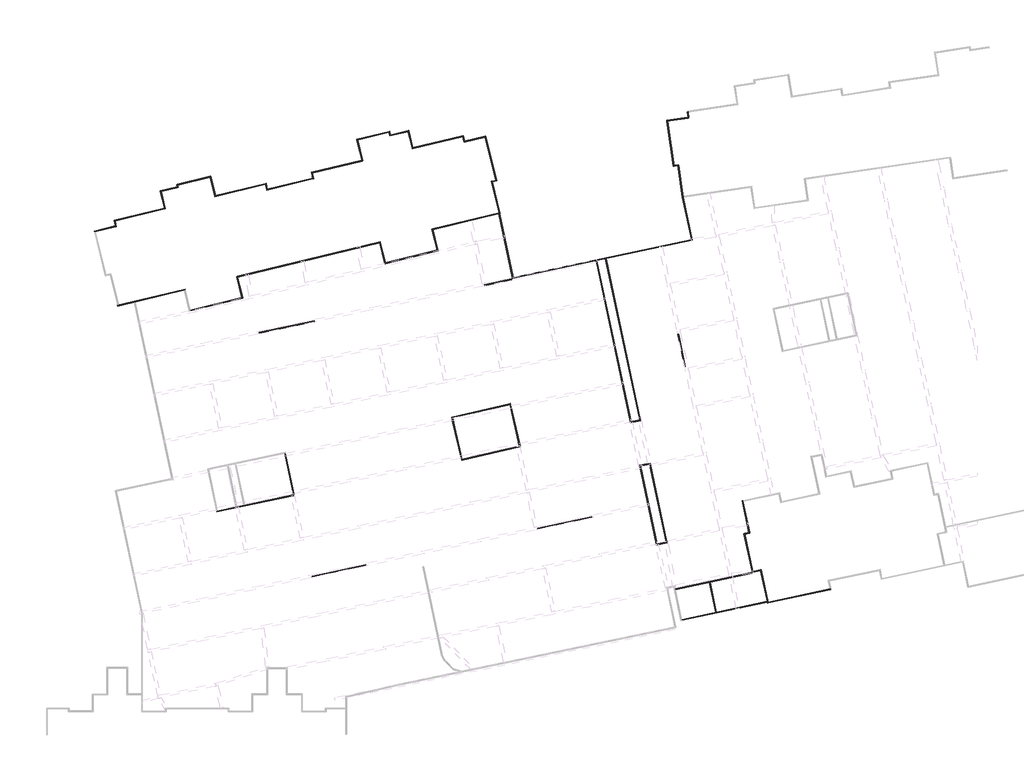
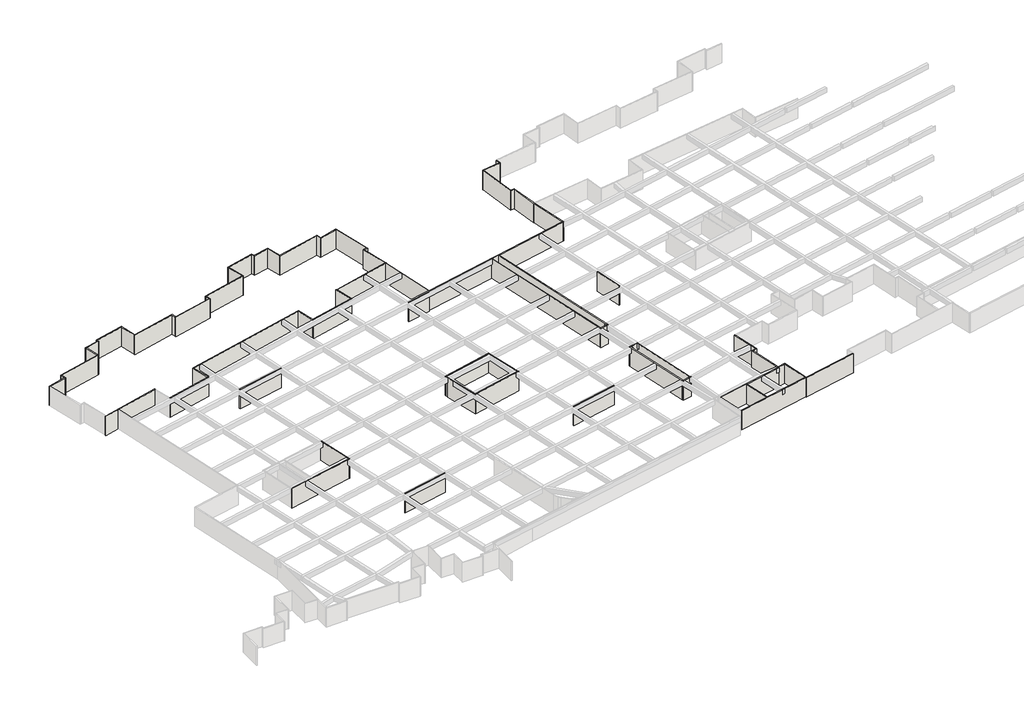
# One storey, part 2 of 14: 68 walls.
"""IFC4 building model written with IfcOpenShell, lengths in millimetres."""

from ifc_helpers import new_model, si_unit, origin, origin_with_axes, place, context, project, spatial, polyline, outline, extrude, faceted_brep, element, save

model = new_model("IFC4")

# Units and contexts
model_context = context("Model", 3, world=origin())
ifc_project = project(units=[si_unit("LENGTHUNIT", "METRE", prefix="MILLI")], contexts=[model_context])

# Site, building, storey
site = spatial("IfcSite", under=ifc_project)
building = spatial("IfcBuilding", under=site)
storey = spatial("IfcBuildingStorey", under=building, Name="户型图", Elevation=0.0)

# Walls
placement = place(None, origin())
element("IfcWall", 1, ObjectType="所有墙体", at=placement, inside=storey, context=model_context, shape_type="Brep", body=[
    faceted_brep([(-247680.1247195, -194264.9696016, 0.0), (-247705.0741224, -194147.5918895, 0.0), (-248661.634697, -189647.3282085, 0.0), (-248661.634697, -189647.3282085, 3300.0), (-247705.0741224, -194147.5918895, 3300.0), (-247680.1247195, -194264.9696016, 3300.0), (-247797.5024316, -194289.9190045, 0.0), (-247797.5024316, -194289.9190045, 3300.0), (-247821.8102949, -194175.5594989, 3300.0), (-247846.7596978, -194058.1817868, 3300.0), (-248754.0630062, -189789.6553235, 3300.0), (-248779.0124091, -189672.2776114, 3300.0), (-248779.0124091, -189672.2776114, 0.0), (-248754.0630062, -189789.6553235, 0.0), (-247846.7596978, -194058.1817868, 0.0), (-247821.8102949, -194175.5594989, 0.0)], [[[0, 1, 2, 3, 4, 5]], [[6, 7, 8, 9, 10, 11, 12, 13, 14, 15]], [[2, 1, 0, 6, 15, 14, 13, 12]], [[5, 4, 3, 11, 10, 9, 8, 7]], [[3, 2, 12, 11]], [[0, 5, 7, 6]]]),
])
element("IfcWall", 2, ObjectType="所有墙体", at=placement, inside=storey, context=model_context, shape_type="Brep", body=[
    faceted_brep([(-248779.0124091, -189672.2776114, 0.0), (-249835.4118179, -189896.8222375, 0.0), (-249952.78953, -189921.7716404, 0.0), (-249952.78953, -189921.7716404, 3300.0), (-249835.4118179, -189896.8222375, 3300.0), (-248779.0124091, -189672.2776114, 3300.0), (-248754.0630062, -189789.6553235, 0.0), (-248754.0630062, -189789.6553235, 3300.0), (-249927.8401271, -190039.1493525, 3300.0), (-249927.8401271, -190039.1493525, 0.0), (-249932.532469, -190017.0736194, 0.0), (-249932.532469, -190017.0736194, 3300.0)], [[[0, 1, 2, 3, 4, 5]], [[6, 7, 8, 9]], [[2, 1, 0, 6, 9, 10]], [[5, 4, 3, 11, 8, 7]], [[0, 5, 7, 6]], [[3, 2, 10, 9, 8, 11]]]),
])
element("IfcWall", 3, ObjectType="所有墙体", at=placement, inside=storey, context=model_context, shape_type="Brep", body=[
    faceted_brep([(-249835.4118179, -189896.8222375, 0.0), (-250933.1855454, -184732.2029056, 0.0), (-250958.1349483, -184614.8251935, 0.0), (-250958.1349483, -184614.8251935, 3300.0), (-250933.1855454, -184732.2029056, 3300.0), (-249835.4118179, -189896.8222375, 3300.0), (-249952.78953, -189921.7716404, 0.0), (-249952.78953, -189921.7716404, 3300.0), (-251075.5126604, -184639.7745964, 3300.0), (-251075.5126604, -184639.7745964, 0.0)], [[[0, 1, 2, 3, 4, 5]], [[6, 7, 8, 9]], [[2, 1, 0, 6, 9]], [[5, 4, 3, 8, 7]], [[0, 5, 7, 6]], [[3, 2, 9, 8]]]),
])
element("IfcWall", 4, ObjectType="所有墙体", at=placement, inside=storey, context=model_context, shape_type="Brep", body=[
    faceted_brep([(-250933.1855454, -184732.2029056, 0.0), (-250248.4822249, -184586.6647221, 0.0), (-250248.4822249, -184586.6647221, 3300.0), (-250933.1855454, -184732.2029056, 3300.0), (-250958.1349483, -184614.8251935, 0.0), (-250958.1349483, -184614.8251935, 3300.0), (-250390.8093399, -184494.2364129, 3300.0), (-250273.4316278, -184469.28701, 3300.0), (-250273.4316278, -184469.28701, 0.0), (-250390.8093399, -184494.2364129, 0.0)], [[[0, 1, 2, 3]], [[4, 5, 6, 7, 8, 9]], [[1, 0, 4, 9, 8]], [[3, 2, 7, 6, 5]], [[0, 3, 5, 4]], [[2, 1, 8, 7]]]),
])
element("IfcWall", 5, ObjectType="所有墙体", at=placement, inside=storey, context=model_context, shape_type="Brep", body=[
    faceted_brep([(-250273.4316278, -184469.28701, 0.0), (-251184.7932427, -180181.6677158, 0.0), (-251209.7426456, -180064.2900037, 0.0), (-251209.7426456, -180064.2900037, 3300.0), (-251184.7932427, -180181.6677158, 3300.0), (-250273.4316278, -184469.28701, 3300.0), (-250390.8093399, -184494.2364129, 0.0), (-250390.8093399, -184494.2364129, 3300.0), (-251327.1203577, -180089.2394066, 3300.0), (-251327.1203577, -180089.2394066, 0.0)], [[[0, 1, 2, 3, 4, 5]], [[6, 7, 8, 9]], [[2, 1, 0, 6, 9]], [[5, 4, 3, 8, 7]], [[0, 5, 7, 6]], [[3, 2, 9, 8]]]),
])
element("IfcWall", 6, ObjectType="所有墙体", at=placement, inside=storey, context=model_context, shape_type="SweptSolid", body=[
    extrude(outline(polyline([(-247705.0741224, -194147.5918895), (-239110.0463222, -192320.6623328), (-239085.0969193, -192438.0400449), (-247680.1247195, -194264.9696016), (-247705.0741224, -194147.5918895)])), origin_with_axes(), (0.0, 0.0, 1.0), 3300.0),
])
element("IfcWall", 7, ObjectType="所有墙体", at=placement, inside=storey, context=model_context, shape_type="Brep", body=[
    faceted_brep([(-258948.9869471, -126119.2790497, 0.0), (-258844.3642989, -126831.6371769, 0.0), (-258826.9271908, -126950.3635315, 0.0), (-258826.9271908, -126950.3635315, 3300.0), (-258844.3642989, -126831.6371769, 3300.0), (-258948.9869471, -126119.2790497, 3300.0), (-258830.2605925, -126101.8419416, 0.0), (-258830.2605925, -126101.8419416, 3300.0), (-258708.2008363, -126932.9264234, 3300.0), (-258708.2008363, -126932.9264234, 0.0)], [[[0, 1, 2, 3, 4, 5]], [[6, 7, 8, 9]], [[2, 1, 0, 6, 9]], [[5, 4, 3, 8, 7]], [[0, 5, 7, 6]], [[3, 2, 9, 8]]]),
])
element("IfcWall", 8, ObjectType="所有墙体", at=placement, inside=storey, context=model_context, shape_type="Brep", body=[
    faceted_brep([(-258844.3642989, -126831.6371769, 0.0), (-261812.5231625, -127267.5648778, 0.0), (-261812.5231625, -127267.5648778, 3300.0), (-258844.3642989, -126831.6371769, 3300.0), (-258826.9271908, -126950.3635315, 0.0), (-258826.9271908, -126950.3635315, 3300.0), (-261676.3596999, -127368.8541243, 3300.0), (-261795.0860545, -127386.2912323, 3300.0), (-261795.0860545, -127386.2912323, 0.0), (-261676.3596999, -127368.8541243, 0.0)], [[[0, 1, 2, 3]], [[4, 5, 6, 7, 8, 9]], [[1, 0, 4, 9, 8]], [[3, 2, 7, 6, 5]], [[0, 3, 5, 4]], [[2, 1, 8, 7]]]),
])
element("IfcWall", 9, ObjectType="所有墙体", at=placement, inside=storey, context=model_context, shape_type="Brep", body=[
    faceted_brep([(-261795.0860545, -127386.2912323, 0.0), (-260879.6378827, -133619.4248459, 0.0), (-260879.6378827, -133619.4248459, 3300.0), (-261795.0860545, -127386.2912323, 3300.0), (-261676.3596999, -127368.8541243, 0.0), (-261676.3596999, -127368.8541243, 3300.0), (-260778.3486362, -133483.2613833, 3300.0), (-260760.9115282, -133601.9877379, 3300.0), (-260760.9115282, -133601.9877379, 0.0), (-260778.3486362, -133483.2613833, 0.0)], [[[0, 1, 2, 3]], [[4, 5, 6, 7, 8, 9]], [[1, 0, 4, 9, 8]], [[3, 2, 7, 6, 5]], [[0, 3, 5, 4]], [[2, 1, 8, 7]]]),
])
element("IfcWall", 10, ObjectType="所有墙体", at=placement, inside=storey, context=model_context, shape_type="Brep", body=[
    faceted_brep([(-260760.9115282, -133601.9877379, 0.0), (-260267.9501372, -133529.5874602, 0.0), (-260149.2237827, -133512.1503522, 0.0), (-260149.2237827, -133512.1503522, 3300.0), (-260267.9501372, -133529.5874602, 3300.0), (-260760.9115282, -133601.9877379, 3300.0), (-260778.3486362, -133483.2613833, 0.0), (-260778.3486362, -133483.2613833, 3300.0), (-260166.6608907, -133393.4239977, 3300.0), (-260166.6608907, -133393.4239977, 0.0)], [[[0, 1, 2, 3, 4, 5]], [[6, 7, 8, 9]], [[2, 1, 0, 6, 9]], [[5, 4, 3, 8, 7]], [[0, 5, 7, 6]], [[3, 2, 9, 8]]]),
])
element("IfcWall", 11, ObjectType="所有墙体", at=placement, inside=storey, context=model_context, shape_type="Brep", body=[
    faceted_brep([(-260267.9501372, -133529.5874602, 0.0), (-259616.5559691, -137964.8214911, 0.0), (-259616.5559691, -137964.8214911, 3300.0), (-260267.9501372, -133529.5874602, 3300.0), (-260149.2237827, -133512.1503522, 0.0), (-260149.2237827, -133512.1503522, 3300.0), (-259515.2667226, -137828.6580286, 3300.0), (-259497.8296146, -137947.3843831, 3300.0), (-259497.8296146, -137947.3843831, 0.0), (-259515.2667226, -137828.6580286, 0.0), (-259612.8948547, -137964.2837904, 0.0), (-259612.8948547, -137964.2837904, 3300.0)], [[[0, 1, 2, 3]], [[4, 5, 6, 7, 8, 9]], [[1, 0, 4, 9, 8, 10]], [[3, 2, 11, 7, 6, 5]], [[0, 3, 5, 4]], [[2, 1, 10, 8, 7, 11]]]),
])
element("IfcWall", 12, ObjectType="所有墙体", at=placement, inside=storey, context=model_context, shape_type="Brep", body=[
    faceted_brep([(-338038.3860994, -153082.5880427, 0.0), (-335711.2604986, -152517.7311777, 0.0), (-335594.5985969, -152489.4141517, 0.0), (-328767.5797313, -150832.3104387, 0.0), (-328650.9658147, -150804.0050601, 0.0), (-328650.9658147, -150804.0050601, 3300.0), (-328767.5797313, -150832.3104387, 3300.0), (-335594.5985969, -152489.4141517, 3300.0), (-335711.2604986, -152517.7311777, 3300.0), (-338038.3860994, -153082.5880427, 3300.0), (-338066.691478, -152965.9741261, 0.0), (-338066.691478, -152965.9741261, 3300.0), (-338027.8201762, -152956.5390008, 3300.0), (-337911.2062596, -152928.2336221, 3300.0), (-328679.2711934, -150687.3911435, 3300.0), (-328679.2711934, -150687.3911435, 0.0), (-337911.2062596, -152928.2336221, 0.0), (-338027.8201762, -152956.5390008, 0.0)], [[[0, 1, 2, 3, 4, 5, 6, 7, 8, 9]], [[10, 11, 12, 13, 14, 15, 16, 17]], [[4, 3, 2, 1, 0, 10, 17, 16, 15]], [[9, 8, 7, 6, 5, 14, 13, 12, 11]], [[0, 9, 11, 10]], [[5, 4, 15, 14]]]),
])
element("IfcWall", 13, ObjectType="所有墙体", at=placement, inside=storey, context=model_context, shape_type="Brep", body=[
    faceted_brep([(-327943.3313501, -153719.3529662, 0.0), (-320654.9615625, -151950.2667992, 0.0), (-320654.9615625, -151950.2667992, 3300.0), (-327943.3313501, -153719.3529662, 3300.0), (-327971.6367288, -153602.7390496, 0.0), (-327971.6367288, -153602.7390496, 3300.0), (-320799.8808577, -151861.9582613, 3300.0), (-320683.2669411, -151833.6528826, 3300.0), (-320683.2669411, -151833.6528826, 0.0), (-320799.8808577, -151861.9582613, 0.0)], [[[0, 1, 2, 3]], [[4, 5, 6, 7, 8, 9]], [[1, 0, 4, 9, 8]], [[3, 2, 7, 6, 5]], [[0, 3, 5, 4]], [[2, 1, 8, 7]]]),
])
element("IfcWall", 14, ObjectType="所有墙体", at=placement, inside=storey, context=model_context, shape_type="Brep", body=[
    faceted_brep([(-320683.2669411, -151833.6528826, 0.0), (-321362.5960271, -149034.9188931, 0.0), (-321390.9014057, -148918.3049765, 0.0), (-321390.9014057, -148918.3049765, 3300.0), (-321362.5960271, -149034.9188931, 3300.0), (-320683.2669411, -151833.6528826, 3300.0), (-320799.8808577, -151861.9582613, 0.0), (-320799.8808577, -151861.9582613, 3300.0), (-321507.5153223, -148946.6103552, 3300.0), (-321507.5153223, -148946.6103552, 0.0)], [[[0, 1, 2, 3, 4, 5]], [[6, 7, 8, 9]], [[2, 1, 0, 6, 9]], [[5, 4, 3, 8, 7]], [[0, 5, 7, 6]], [[3, 2, 9, 8]]]),
])
element("IfcWall", 15, ObjectType="所有墙体", at=placement, inside=storey, context=model_context, shape_type="Brep", body=[
    faceted_brep([(-321362.5960271, -149034.9188931, 0.0), (-301654.8441261, -144251.3098988, 0.0), (-301538.2302095, -144223.0045201, 0.0), (-301538.2302095, -144223.0045201, 3300.0), (-301654.8441261, -144251.3098988, 3300.0), (-321362.5960271, -149034.9188931, 3300.0), (-321390.9014057, -148918.3049765, 0.0), (-321390.9014057, -148918.3049765, 3300.0), (-301566.5355882, -144106.3906035, 3300.0), (-301566.5355882, -144106.3906035, 0.0)], [[[0, 1, 2, 3, 4, 5]], [[6, 7, 8, 9]], [[2, 1, 0, 6, 9]], [[5, 4, 3, 8, 7]], [[0, 5, 7, 6]], [[3, 2, 9, 8]]]),
])
element("IfcWall", 16, ObjectType="所有墙体", at=placement, inside=storey, context=model_context, shape_type="Brep", body=[
    faceted_brep([(-301654.8441261, -144251.3098988, 0.0), (-300947.2096643, -147166.6577934, 0.0), (-300947.2096643, -147166.6577934, 3300.0), (-301654.8441261, -144251.3098988, 3300.0), (-301538.2302095, -144223.0045201, 0.0), (-301538.2302095, -144223.0045201, 3300.0), (-300858.9011264, -147021.7384982, 3300.0), (-300830.5957477, -147138.3524148, 3300.0), (-300830.5957477, -147138.3524148, 0.0), (-300858.9011264, -147021.7384982, 0.0)], [[[0, 1, 2, 3]], [[4, 5, 6, 7, 8, 9]], [[1, 0, 4, 9, 8]], [[3, 2, 7, 6, 5]], [[0, 3, 5, 4]], [[2, 1, 8, 7]]]),
])
element("IfcWall", 17, ObjectType="所有墙体", at=placement, inside=storey, context=model_context, shape_type="Brep", body=[
    faceted_brep([(-300830.5957477, -147138.3524148, 0.0), (-293542.2259606, -145369.2662479, 0.0), (-293542.2259606, -145369.2662479, 3300.0), (-300830.5957477, -147138.3524148, 3300.0), (-300858.9011264, -147021.7384982, 0.0), (-300858.9011264, -147021.7384982, 3300.0), (-293687.1452559, -145280.95771, 3300.0), (-293570.5313393, -145252.6523314, 3300.0), (-293570.5313393, -145252.6523314, 0.0), (-293687.1452559, -145280.95771, 0.0)], [[[0, 1, 2, 3]], [[4, 5, 6, 7, 8, 9]], [[1, 0, 4, 9, 8]], [[3, 2, 7, 6, 5]], [[0, 3, 5, 4]], [[2, 1, 8, 7]]]),
])
element("IfcWall", 18, ObjectType="所有墙体", at=placement, inside=storey, context=model_context, shape_type="Brep", body=[
    faceted_brep([(-293570.5313393, -145252.6523314, 0.0), (-294249.8604225, -142453.9183533, 0.0), (-294278.1658011, -142337.3044367, 0.0), (-294278.1658011, -142337.3044367, 3300.0), (-294249.8604225, -142453.9183533, 3300.0), (-293570.5313393, -145252.6523314, 3300.0), (-293687.1452559, -145280.95771, 0.0), (-293687.1452559, -145280.95771, 3300.0), (-294394.7797177, -142365.6098154, 3300.0), (-294394.7797177, -142365.6098154, 0.0)], [[[0, 1, 2, 3, 4, 5]], [[6, 7, 8, 9]], [[2, 1, 0, 6, 9]], [[5, 4, 3, 8, 7]], [[0, 5, 7, 6]], [[3, 2, 9, 8]]]),
])
element("IfcWall", 19, ObjectType="所有墙体", at=placement, inside=storey, context=model_context, shape_type="Brep", body=[
    faceted_brep([(-294249.8604225, -142453.9183533, 0.0), (-285098.2083864, -140232.5627561, 0.0), (-284981.5464847, -140204.2457302, 0.0), (-284920.7470789, -140189.4880558, 0.0), (-284920.7470789, -140189.4880558, 3300.0), (-284981.5464847, -140204.2457302, 3300.0), (-285098.2083864, -140232.5627561, 3300.0), (-294249.8604225, -142453.9183533, 3300.0), (-294278.1658011, -142337.3044367, 0.0), (-294278.1658011, -142337.3044367, 3300.0), (-285065.6663741, -140101.1795179, 3300.0), (-284949.0524575, -140072.8741393, 3300.0), (-284949.0524575, -140072.8741393, 0.0), (-285065.6663741, -140101.1795179, 0.0)], [[[0, 1, 2, 3, 4, 5, 6, 7]], [[8, 9, 10, 11, 12, 13]], [[3, 2, 1, 0, 8, 13, 12]], [[7, 6, 5, 4, 11, 10, 9]], [[0, 7, 9, 8]], [[4, 3, 12, 11]]]),
])
element("IfcWall", 20, ObjectType="所有墙体", at=placement, inside=storey, context=model_context, shape_type="Brep", body=[
    faceted_brep([(-284949.0524575, -140072.8741393, 0.0), (-285982.1987791, -135816.4661828, 0.0), (-286010.5041578, -135699.8522663, 0.0), (-286010.5041578, -135699.8522663, 3300.0), (-285982.1987791, -135816.4661828, 3300.0), (-284949.0524575, -140072.8741393, 3300.0), (-285065.6663741, -140101.1795179, 0.0), (-285065.6663741, -140101.1795179, 3300.0), (-286127.1180744, -135728.1576449, 3300.0), (-286127.1180744, -135728.1576449, 0.0)], [[[0, 1, 2, 3, 4, 5]], [[6, 7, 8, 9]], [[2, 1, 0, 6, 9]], [[5, 4, 3, 8, 7]], [[0, 5, 7, 6]], [[3, 2, 9, 8]]]),
])
element("IfcWall", 21, ObjectType="所有墙体", at=placement, inside=storey, context=model_context, shape_type="Brep", body=[
    faceted_brep([(-285982.1987791, -135816.4661828, 0.0), (-285399.1292138, -135674.9392938, 0.0), (-285399.1292138, -135674.9392938, 3300.0), (-285982.1987791, -135816.4661828, 3300.0), (-286010.5041578, -135699.8522663, 0.0), (-286010.5041578, -135699.8522663, 3300.0), (-285544.0485091, -135586.6307559, 3300.0), (-285427.4345925, -135558.3253772, 3300.0), (-285427.4345925, -135558.3253772, 0.0), (-285544.0485091, -135586.6307559, 0.0)], [[[0, 1, 2, 3]], [[4, 5, 6, 7, 8, 9]], [[1, 0, 4, 9, 8]], [[3, 2, 7, 6, 5]], [[0, 3, 5, 4]], [[2, 1, 8, 7]]]),
])
element("IfcWall", 22, ObjectType="所有墙体", at=placement, inside=storey, context=model_context, shape_type="Brep", body=[
    faceted_brep([(-285427.4345925, -135558.3253772, 0.0), (-286913.4669714, -129436.0947611, 0.0), (-286913.4669714, -129436.0947611, 3300.0), (-285427.4345925, -135558.3253772, 3300.0), (-285544.0485091, -135586.6307559, 0.0), (-285544.0485091, -135586.6307559, 3300.0), (-287001.7755093, -129581.0140564, 3300.0), (-287030.080888, -129464.4001398, 3300.0), (-287030.080888, -129464.4001398, 0.0), (-287001.7755093, -129581.0140564, 0.0)], [[[0, 1, 2, 3]], [[4, 5, 6, 7, 8, 9]], [[1, 0, 4, 9, 8]], [[3, 2, 7, 6, 5]], [[0, 3, 5, 4]], [[2, 1, 8, 7]]]),
])
element("IfcWall", 23, ObjectType="所有墙体", at=placement, inside=storey, context=model_context, shape_type="Brep", body=[
    faceted_brep([(-287030.080888, -129464.4001398, 0.0), (-289828.8148854, -130143.7292277, 0.0), (-289945.428802, -130172.0346063, 0.0), (-289945.428802, -130172.0346063, 3300.0), (-289828.8148854, -130143.7292277, 3300.0), (-287030.080888, -129464.4001398, 3300.0), (-287001.7755093, -129581.0140564, 0.0), (-287001.7755093, -129581.0140564, 3300.0), (-289917.1234233, -130288.6485229, 3300.0), (-289917.1234233, -130288.6485229, 0.0)], [[[0, 1, 2, 3, 4, 5]], [[6, 7, 8, 9]], [[2, 1, 0, 6, 9]], [[5, 4, 3, 8, 7]], [[0, 5, 7, 6]], [[3, 2, 9, 8]]]),
])
element("IfcWall", 24, ObjectType="所有墙体", at=placement, inside=storey, context=model_context, shape_type="Brep", body=[
    faceted_brep([(-289828.8148854, -130143.7292277, 0.0), (-290017.5174109, -129366.3031131, 0.0), (-290017.5174109, -129366.3031131, 3300.0), (-289828.8148854, -130143.7292277, 3300.0), (-289945.428802, -130172.0346063, 0.0), (-289945.428802, -130172.0346063, 3300.0), (-290105.8259488, -129511.2224083, 3300.0), (-290134.1313274, -129394.6084918, 3300.0), (-290134.1313274, -129394.6084918, 0.0), (-290105.8259488, -129511.2224083, 0.0)], [[[0, 1, 2, 3]], [[4, 5, 6, 7, 8, 9]], [[1, 0, 4, 9, 8]], [[3, 2, 7, 6, 5]], [[0, 3, 5, 4]], [[2, 1, 8, 7]]]),
])
element("IfcWall", 25, ObjectType="所有墙体", at=placement, inside=storey, context=model_context, shape_type="Brep", body=[
    faceted_brep([(-290134.1313274, -129394.6084918, 0.0), (-297038.6469685, -131070.5227862, 0.0), (-297155.260885, -131098.8281648, 0.0), (-297155.260885, -131098.8281648, 3300.0), (-297038.6469685, -131070.5227862, 3300.0), (-290134.1313274, -129394.6084918, 3300.0), (-290105.8259488, -129511.2224083, 0.0), (-290105.8259488, -129511.2224083, 3300.0), (-297126.9555064, -131215.4420814, 3300.0), (-297126.9555064, -131215.4420814, 0.0)], [[[0, 1, 2, 3, 4, 5]], [[6, 7, 8, 9]], [[2, 1, 0, 6, 9]], [[5, 4, 3, 8, 7]], [[0, 5, 7, 6]], [[3, 2, 9, 8]]]),
])
element("IfcWall", 26, ObjectType="所有墙体", at=placement, inside=storey, context=model_context, shape_type="Brep", body=[
    faceted_brep([(-297038.6469685, -131070.5227862, 0.0), (-297622.4454055, -128665.3607481, 0.0), (-297622.4454055, -128665.3607481, 3300.0), (-297038.6469685, -131070.5227862, 3300.0), (-297155.260885, -131098.8281648, 0.0), (-297155.260885, -131098.8281648, 3300.0), (-297710.7539434, -128810.2800434, 3300.0), (-297739.0593221, -128693.6661268, 3300.0), (-297739.0593221, -128693.6661268, 0.0), (-297710.7539434, -128810.2800434, 0.0)], [[[0, 1, 2, 3]], [[4, 5, 6, 7, 8, 9]], [[1, 0, 4, 9, 8]], [[3, 2, 7, 6, 5]], [[0, 3, 5, 4]], [[2, 1, 8, 7]]]),
])
element("IfcWall", 27, ObjectType="所有墙体", at=placement, inside=storey, context=model_context, shape_type="Brep", body=[
    faceted_brep([(-297739.0593221, -128693.6661268, 0.0), (-300149.0802646, -129278.6439525, 0.0), (-300265.6941812, -129306.9493312, 0.0), (-300265.6941812, -129306.9493312, 3300.0), (-300149.0802646, -129278.6439525, 3300.0), (-297739.0593221, -128693.6661268, 3300.0), (-297710.7539434, -128810.2800434, 0.0), (-297710.7539434, -128810.2800434, 3300.0), (-300237.3888025, -129423.5632478, 3300.0), (-300237.3888025, -129423.5632478, 0.0)], [[[0, 1, 2, 3, 4, 5]], [[6, 7, 8, 9]], [[2, 1, 0, 6, 9]], [[5, 4, 3, 8, 7]], [[0, 5, 7, 6]], [[3, 2, 9, 8]]]),
])
element("IfcWall", 28, ObjectType="所有墙体", at=placement, inside=storey, context=model_context, shape_type="Brep", body=[
    faceted_brep([(-300149.0802646, -129278.6439525, 0.0), (-300267.0193424, -128792.7526335, 0.0), (-300267.0193424, -128792.7526335, 3300.0), (-300149.0802646, -129278.6439525, 3300.0), (-300265.6941812, -129306.9493312, 0.0), (-300265.6941812, -129306.9493312, 3300.0), (-300355.3278803, -128937.6719287, 3300.0), (-300383.633259, -128821.0580121, 3300.0), (-300383.633259, -128821.0580121, 0.0), (-300355.3278803, -128937.6719287, 0.0)], [[[0, 1, 2, 3]], [[4, 5, 6, 7, 8, 9]], [[1, 0, 4, 9, 8]], [[3, 2, 7, 6, 5]], [[0, 3, 5, 4]], [[2, 1, 8, 7]]]),
])
element("IfcWall", 29, ObjectType="所有墙体", at=placement, inside=storey, context=model_context, shape_type="Brep", body=[
    faceted_brep([(-300383.633259, -128821.0580121, 0.0), (-304829.5388252, -129900.200573, 0.0), (-304829.5388252, -129900.200573, 3300.0), (-300383.633259, -128821.0580121, 3300.0), (-300355.3278803, -128937.6719287, 0.0), (-300355.3278803, -128937.6719287, 3300.0), (-304684.61953, -129988.5091109, 3300.0), (-304801.2334465, -130016.8144895, 3300.0), (-304801.2334465, -130016.8144895, 0.0), (-304684.61953, -129988.5091109, 0.0)], [[[0, 1, 2, 3]], [[4, 5, 6, 7, 8, 9]], [[1, 0, 4, 9, 8]], [[3, 2, 7, 6, 5]], [[0, 3, 5, 4]], [[2, 1, 8, 7]]]),
])
element("IfcWall", 30, ObjectType="所有墙体", at=placement, inside=storey, context=model_context, shape_type="Brep", body=[
    faceted_brep([(-304801.2334465, -130016.8144895, 0.0), (-304127.8013104, -132791.2539301, 0.0), (-304099.4959317, -132907.8678466, 0.0), (-304099.4959317, -132907.8678466, 3300.0), (-304127.8013104, -132791.2539301, 3300.0), (-304801.2334465, -130016.8144895, 3300.0), (-304684.61953, -129988.5091109, 0.0), (-304684.61953, -129988.5091109, 3300.0), (-303982.8820151, -132879.562468, 3300.0), (-303982.8820151, -132879.562468, 0.0)], [[[0, 1, 2, 3, 4, 5]], [[6, 7, 8, 9]], [[2, 1, 0, 6, 9]], [[5, 4, 3, 8, 7]], [[0, 5, 7, 6]], [[3, 2, 9, 8]]]),
])
element("IfcWall", 31, ObjectType="所有墙体", at=placement, inside=storey, context=model_context, shape_type="Brep", body=[
    faceted_brep([(-304127.8013104, -132791.2539301, 0.0), (-311124.6363112, -134489.5766515, 0.0), (-311124.6363112, -134489.5766515, 3300.0), (-304127.8013104, -132791.2539301, 3300.0), (-304099.4959317, -132907.8678466, 0.0), (-304099.4959317, -132907.8678466, 3300.0), (-310979.7170159, -134577.8851894, 3300.0), (-311096.3309325, -134606.1905681, 3300.0), (-311096.3309325, -134606.1905681, 0.0), (-310979.7170159, -134577.8851894, 0.0)], [[[0, 1, 2, 3]], [[4, 5, 6, 7, 8, 9]], [[1, 0, 4, 9, 8]], [[3, 2, 7, 6, 5]], [[0, 3, 5, 4]], [[2, 1, 8, 7]]]),
])
element("IfcWall", 32, ObjectType="所有墙体", at=placement, inside=storey, context=model_context, shape_type="Brep", body=[
    faceted_brep([(-311096.3309325, -134606.1905681, 0.0), (-310935.933787, -135267.0027608, 0.0), (-310907.6284084, -135383.6166773, 0.0), (-310907.6284084, -135383.6166773, 3300.0), (-310935.933787, -135267.0027608, 3300.0), (-311096.3309325, -134606.1905681, 3300.0), (-310979.7170159, -134577.8851894, 0.0), (-310979.7170159, -134577.8851894, 3300.0), (-310791.0144918, -135355.3112987, 3300.0), (-310791.0144918, -135355.3112987, 0.0)], [[[0, 1, 2, 3, 4, 5]], [[6, 7, 8, 9]], [[2, 1, 0, 6, 9]], [[5, 4, 3, 8, 7]], [[0, 5, 7, 6]], [[3, 2, 9, 8]]]),
])
element("IfcWall", 33, ObjectType="所有墙体", at=placement, inside=storey, context=model_context, shape_type="Brep", body=[
    faceted_brep([(-310935.933787, -135267.0027608, 0.0), (-317233.0852904, -136795.4932107, 0.0), (-317349.699207, -136823.7985893, 0.0), (-317349.699207, -136823.7985893, 3300.0), (-317233.0852904, -136795.4932107, 3300.0), (-310935.933787, -135267.0027608, 3300.0), (-310907.6284084, -135383.6166773, 0.0), (-310907.6284084, -135383.6166773, 3300.0), (-317321.3938283, -136940.4125059, 3300.0), (-317321.3938283, -136940.4125059, 0.0)], [[[0, 1, 2, 3, 4, 5]], [[6, 7, 8, 9]], [[2, 1, 0, 6, 9]], [[5, 4, 3, 8, 7]], [[0, 5, 7, 6]], [[3, 2, 9, 8]]]),
])
element("IfcWall", 34, ObjectType="所有墙体", at=placement, inside=storey, context=model_context, shape_type="Brep", body=[
    faceted_brep([(-317233.0852904, -136795.4932107, 0.0), (-317421.7878145, -136018.0671014, 0.0), (-317421.7878145, -136018.0671014, 3300.0), (-317233.0852904, -136795.4932107, 3300.0), (-317349.699207, -136823.7985893, 0.0), (-317349.699207, -136823.7985893, 3300.0), (-317510.0963524, -136162.9863966, 3300.0), (-317538.4017311, -136046.3724801, 3300.0), (-317538.4017311, -136046.3724801, 0.0), (-317510.0963524, -136162.9863966, 0.0)], [[[0, 1, 2, 3]], [[4, 5, 6, 7, 8, 9]], [[1, 0, 4, 9, 8]], [[3, 2, 7, 6, 5]], [[0, 3, 5, 4]], [[2, 1, 8, 7]]]),
])
element("IfcWall", 35, ObjectType="所有墙体", at=placement, inside=storey, context=model_context, shape_type="Brep", body=[
    faceted_brep([(-317538.4017311, -136046.3724801, 0.0), (-324442.9173664, -137722.2867731, 0.0), (-324559.531283, -137750.5921518, 0.0), (-324559.531283, -137750.5921518, 3300.0), (-324442.9173664, -137722.2867731, 3300.0), (-317538.4017311, -136046.3724801, 3300.0), (-317510.0963524, -136162.9863966, 0.0), (-317510.0963524, -136162.9863966, 3300.0), (-324531.2259043, -137867.2060683, 3300.0), (-324531.2259043, -137867.2060683, 0.0)], [[[0, 1, 2, 3, 4, 5]], [[6, 7, 8, 9]], [[2, 1, 0, 6, 9]], [[5, 4, 3, 8, 7]], [[0, 5, 7, 6]], [[3, 2, 9, 8]]]),
])
element("IfcWall", 36, ObjectType="所有墙体", at=placement, inside=storey, context=model_context, shape_type="Brep", body=[
    faceted_brep([(-324442.9173664, -137722.2867731, 0.0), (-325097.4847175, -135025.5674191, 0.0), (-325097.4847175, -135025.5674191, 3300.0), (-324442.9173664, -137722.2867731, 3300.0), (-324559.531283, -137750.5921518, 0.0), (-324559.531283, -137750.5921518, 3300.0), (-325185.7932554, -135170.4867144, 3300.0), (-325214.098634, -135053.8727978, 3300.0), (-325214.098634, -135053.8727978, 0.0), (-325185.7932554, -135170.4867144, 0.0)], [[[0, 1, 2, 3]], [[4, 5, 6, 7, 8, 9]], [[1, 0, 4, 9, 8]], [[3, 2, 7, 6, 5]], [[0, 3, 5, 4]], [[2, 1, 8, 7]]]),
])
element("IfcWall", 37, ObjectType="所有墙体", at=placement, inside=storey, context=model_context, shape_type="SweptSolid", body=[
    extrude(outline(polyline([(-329737.746821, -136151.8856134), (-325214.098634, -135053.8727978), (-325185.7932554, -135170.4867144), (-329709.4414424, -136268.49953), (-329737.746821, -136151.8856134)])), origin_with_axes(), (0.0, 0.0, 1.0), 3300.0),
])
element("IfcWall", 38, ObjectType="所有墙体", at=placement, inside=storey, context=model_context, shape_type="Brep", body=[
    faceted_brep([(-329854.3607376, -136180.1909921, 0.0), (-329783.5972909, -136471.7257835, 0.0), (-329755.2919123, -136588.3397001, 0.0), (-329755.2919123, -136588.3397001, 3300.0), (-329783.5972909, -136471.7257835, 3300.0), (-329854.3607376, -136180.1909921, 3300.0), (-329737.746821, -136151.8856134, 0.0), (-329737.746821, -136151.8856134, 3300.0), (-329709.4414424, -136268.49953, 3300.0), (-329638.6779957, -136560.0343214, 3300.0), (-329638.6779957, -136560.0343214, 0.0), (-329709.4414424, -136268.49953, 0.0)], [[[0, 1, 2, 3, 4, 5]], [[6, 7, 8, 9, 10, 11]], [[2, 1, 0, 6, 11, 10]], [[5, 4, 3, 9, 8, 7]], [[0, 5, 7, 6]], [[3, 2, 10, 9]]]),
])
element("IfcWall", 39, ObjectType="所有墙体", at=placement, inside=storey, context=model_context, shape_type="Brep", body=[
    faceted_brep([(-329783.5972909, -136471.7257835, 0.0), (-332115.8756224, -137037.8333568, 0.0), (-332115.8756224, -137037.8333568, 3300.0), (-329783.5972909, -136471.7257835, 3300.0), (-329755.2919123, -136588.3397001, 0.0), (-329755.2919123, -136588.3397001, 3300.0), (-331970.9563272, -137126.1418947, 3300.0), (-332087.5702437, -137154.4472734, 3300.0), (-332087.5702437, -137154.4472734, 0.0), (-331970.9563272, -137126.1418947, 0.0)], [[[0, 1, 2, 3]], [[4, 5, 6, 7, 8, 9]], [[1, 0, 4, 9, 8]], [[3, 2, 7, 6, 5]], [[0, 3, 5, 4]], [[2, 1, 8, 7]]]),
])
element("IfcWall", 40, ObjectType="所有墙体", at=placement, inside=storey, context=model_context, shape_type="Brep", body=[
    faceted_brep([(-332087.5702437, -137154.4472734, 0.0), (-331532.071718, -139443.0179193, 0.0), (-331503.7663394, -139559.6318359, 0.0), (-331503.7663394, -139559.6318359, 3300.0), (-331532.071718, -139443.0179193, 3300.0), (-332087.5702437, -137154.4472734, 3300.0), (-331970.9563272, -137126.1418947, 0.0), (-331970.9563272, -137126.1418947, 3300.0), (-331387.1524228, -139531.3264573, 3300.0), (-331387.1524228, -139531.3264573, 0.0)], [[[0, 1, 2, 3, 4, 5]], [[6, 7, 8, 9]], [[2, 1, 0, 6, 9]], [[5, 4, 3, 8, 7]], [[0, 5, 7, 6]], [[3, 2, 9, 8]]]),
])
element("IfcWall", 41, ObjectType="所有墙体", at=placement, inside=storey, context=model_context, shape_type="Brep", body=[
    faceted_brep([(-331532.071718, -139443.0179193, 0.0), (-338528.9067123, -141141.3406392, 0.0), (-338528.9067123, -141141.3406392, 3300.0), (-331532.071718, -139443.0179193, 3300.0), (-331503.7663394, -139559.6318359, 0.0), (-331503.7663394, -139559.6318359, 3300.0), (-338383.9874171, -141229.6491771, 3300.0), (-338500.6013337, -141257.9545558, 3300.0), (-338500.6013337, -141257.9545558, 0.0), (-338383.9874171, -141229.6491771, 0.0)], [[[0, 1, 2, 3]], [[4, 5, 6, 7, 8, 9]], [[1, 0, 4, 9, 8]], [[3, 2, 7, 6, 5]], [[0, 3, 5, 4]], [[2, 1, 8, 7]]]),
])
element("IfcWall", 42, ObjectType="所有墙体", at=placement, inside=storey, context=model_context, shape_type="Brep", body=[
    faceted_brep([(-338500.6013337, -141257.9545558, 0.0), (-338340.2041879, -141918.7667497, 0.0), (-338311.8988092, -142035.3806663, 0.0), (-338311.8988092, -142035.3806663, 3300.0), (-338340.2041879, -141918.7667497, 3300.0), (-338500.6013337, -141257.9545558, 3300.0), (-338383.9874171, -141229.6491771, 0.0), (-338383.9874171, -141229.6491771, 3300.0), (-338195.2848926, -142007.0752876, 3300.0), (-338195.2848926, -142007.0752876, 0.0)], [[[0, 1, 2, 3, 4, 5]], [[6, 7, 8, 9]], [[2, 1, 0, 6, 9]], [[5, 4, 3, 8, 7]], [[0, 5, 7, 6]], [[3, 2, 9, 8]]]),
])
element("IfcWall", 43, ObjectType="所有墙体", at=placement, inside=storey, context=model_context, shape_type="Brep", body=[
    faceted_brep([(-338340.2041879, -141918.7667497, 0.0), (-341255.5521027, -142626.4012164, 0.0), (-341255.5521027, -142626.4012164, 3300.0), (-338340.2041879, -141918.7667497, 3300.0), (-338311.8988092, -142035.3806663, 0.0), (-338311.8988092, -142035.3806663, 3300.0), (-341110.6328075, -142714.7097543, 3300.0), (-341227.2467241, -142743.015133, 3300.0), (-341227.2467241, -142743.015133, 0.0), (-341110.6328075, -142714.7097543, 0.0)], [[[0, 1, 2, 3]], [[4, 5, 6, 7, 8, 9]], [[1, 0, 4, 9, 8]], [[3, 2, 7, 6, 5]], [[0, 3, 5, 4]], [[2, 1, 8, 7]]]),
])
element("IfcWall", 44, ObjectType="所有墙体", at=placement, inside=storey, context=model_context, shape_type="Brep", body=[
    faceted_brep([(-259714.9796049, -196703.5306748, 0.0), (-247821.8102949, -194175.5594989, 0.0), (-247821.8102949, -194175.5594989, 3300.0), (-259714.9796049, -196703.5306748, 3300.0), (-259739.3546313, -196586.0308752, 0.0), (-259739.3546313, -196586.0308752, 3300.0), (-255002.6061391, -195579.2039022, 3300.0), (-254885.228427, -195554.2544993, 3300.0), (-247846.7596978, -194058.1817868, 3300.0), (-247846.7596978, -194058.1817868, 0.0), (-254885.228427, -195554.2544993, 0.0), (-255002.6061391, -195579.2039022, 0.0)], [[[0, 1, 2, 3]], [[4, 5, 6, 7, 8, 9, 10, 11]], [[1, 0, 4, 11, 10, 9]], [[3, 2, 8, 7, 6, 5]], [[0, 3, 5, 4]], [[2, 1, 9, 8]]]),
])
element("IfcWall", 45, ObjectType="所有墙体", at=placement, inside=storey, context=model_context, shape_type="Brep", body=[
    faceted_brep([(-259612.8948547, -137964.2837904, 0.0), (-258368.8135894, -143817.2259697, 0.0), (-258343.8641865, -143934.6036818, 0.0), (-258343.8641865, -143934.6036818, 3300.0), (-258368.8135894, -143817.2259697, 3300.0), (-259612.8948547, -137964.2837904, 3300.0), (-259493.9278671, -137946.8113411, 0.0), (-259493.9278671, -137946.8113411, 3300.0), (-258226.4864744, -143909.6542789, 3300.0), (-258226.4864744, -143909.6542789, 0.0), (-259497.8296146, -137947.3843831, 0.0), (-259497.8296146, -137947.3843831, 3300.0)], [[[0, 1, 2, 3, 4, 5]], [[6, 7, 8, 9]], [[2, 1, 0, 10, 6, 9]], [[5, 4, 3, 8, 7, 11]], [[0, 5, 11, 7, 6, 10]], [[3, 2, 9, 8]]]),
])
element("IfcWall", 46, ObjectType="所有墙体", at=placement, inside=storey, context=model_context, shape_type="Brep", body=[
    faceted_brep([(-258368.8135894, -143817.2259697, 0.0), (-283096.3849359, -149073.2335136, 0.0), (-283213.762648, -149098.1829165, 0.0), (-283213.762648, -149098.1829165, 3300.0), (-283096.3849359, -149073.2335136, 3300.0), (-258368.8135894, -143817.2259697, 3300.0), (-258343.8641865, -143934.6036818, 0.0), (-258343.8641865, -143934.6036818, 3300.0), (-270208.5064079, -146456.5112379, 3300.0), (-270325.88412, -146481.4606408, 3300.0), (-271479.9046193, -146726.7552702, 3300.0), (-271597.2823314, -146751.7046731, 3300.0), (-283188.8132451, -149215.5606286, 3300.0), (-283188.8132451, -149215.5606286, 0.0), (-271597.2823314, -146751.7046731, 0.0), (-271479.9046193, -146726.7552702, 0.0), (-270325.88412, -146481.4606408, 0.0), (-270208.5064079, -146456.5112379, 0.0)], [[[0, 1, 2, 3, 4, 5]], [[6, 7, 8, 9, 10, 11, 12, 13, 14, 15, 16, 17]], [[2, 1, 0, 6, 17, 16, 15, 14, 13]], [[5, 4, 3, 12, 11, 10, 9, 8, 7]], [[0, 5, 7, 6]], [[3, 2, 13, 12]]]),
])
element("IfcWall", 47, ObjectType="所有墙体", at=placement, inside=storey, context=model_context, shape_type="SweptSolid", body=[
    extrude(outline(polyline([(-284981.5464847, -140204.2457302), (-283096.3849359, -149073.2335136), (-283213.762648, -149098.1829165), (-285098.2083864, -140232.5627561), (-284981.5464847, -140204.2457302)])), origin_with_axes(), (0.0, 0.0, 1.0), 3300.0),
])
element("IfcWall", 48, ObjectType="所有墙体", at=placement, inside=storey, context=model_context, shape_type="Brep", body=[
    faceted_brep([(-263221.6377286, -186235.6095743, 0.0), (-261734.8533754, -185919.5838042, 0.0), (-261734.8533754, -185919.5838042, 3300.0), (-263221.6377286, -186235.6095743, 3300.0), (-263246.5871315, -186118.2318622, 0.0), (-263246.5871315, -186118.2318622, 3300.0), (-263129.2094194, -186093.2824593, 3300.0), (-261877.1804904, -185827.1554951, 3300.0), (-261759.8027783, -185802.2060922, 3300.0), (-261759.8027783, -185802.2060922, 0.0), (-261877.1804904, -185827.1554951, 0.0), (-263129.2094194, -186093.2824593, 0.0)], [[[0, 1, 2, 3]], [[4, 5, 6, 7, 8, 9, 10, 11]], [[1, 0, 4, 11, 10, 9]], [[3, 2, 8, 7, 6, 5]], [[2, 1, 9, 8]], [[0, 3, 5, 4]]]),
])
element("IfcWall", 49, ObjectType="所有墙体", at=placement, inside=storey, context=model_context, shape_type="Brep", body=[
    faceted_brep([(-261759.8027783, -185802.2060922, 0.0), (-264088.4137155, -174846.9529639, 0.0), (-264088.4137155, -174846.9529639, 3300.0), (-261759.8027783, -185802.2060922, 3300.0), (-261877.1804904, -185827.1554951, 0.0), (-261877.1804904, -185827.1554951, 3300.0), (-264180.8420247, -174989.2800789, 3300.0), (-264205.7914276, -174871.9023668, 3300.0), (-264205.7914276, -174871.9023668, 0.0), (-264180.8420247, -174989.2800789, 0.0)], [[[0, 1, 2, 3]], [[4, 5, 6, 7, 8, 9]], [[1, 0, 4, 9, 8]], [[3, 2, 7, 6, 5]], [[0, 3, 5, 4]], [[2, 1, 8, 7]]]),
])
element("IfcWall", 50, ObjectType="所有墙体", at=placement, inside=storey, context=model_context, shape_type="Brep", body=[
    faceted_brep([(-264205.7914276, -174871.9023668, 0.0), (-265575.1980686, -175162.978734, 0.0), (-265575.1980686, -175162.978734, 3300.0), (-264205.7914276, -174871.9023668, 3300.0), (-264180.8420247, -174989.2800789, 0.0), (-264180.8420247, -174989.2800789, 3300.0), (-265432.8709536, -175255.4070432, 3300.0), (-265550.2486657, -175280.3564461, 3300.0), (-265550.2486657, -175280.3564461, 0.0), (-265432.8709536, -175255.4070432, 0.0)], [[[0, 1, 2, 3]], [[4, 5, 6, 7, 8, 9]], [[1, 0, 4, 9, 8]], [[3, 2, 7, 6, 5]], [[0, 3, 5, 4]], [[2, 1, 8, 7]]]),
])
element("IfcWall", 51, ObjectType="所有墙体", at=placement, inside=storey, context=model_context, shape_type="SweptSolid", body=[
    extrude(outline(polyline([(-263246.5871315, -186118.2318622), (-265550.2486657, -175280.3564461), (-265432.8709536, -175255.4070432), (-263129.2094194, -186093.2824593), (-263246.5871315, -186118.2318622)])), origin_with_axes(), (0.0, 0.0, 1.0), 3300.0),
])
element("IfcWall", 52, ObjectType="所有墙体", at=placement, inside=storey, context=model_context, shape_type="Brep", body=[
    faceted_brep([(-266813.3081964, -169258.5334313, 0.0), (-265429.6848936, -168939.0988222, 0.0), (-265429.6848936, -168939.0988222, 3300.0), (-266813.3081964, -169258.5334313, 3300.0), (-266838.2613998, -169141.1378393, 0.0), (-266838.2613998, -169141.1378393, 3300.0), (-266721.3191812, -169114.1396008, 3300.0), (-265571.5803156, -168848.7014686, 3300.0), (-265454.638097, -168821.7032301, 3300.0), (-265454.638097, -168821.7032301, 0.0), (-265571.5803156, -168848.7014686, 0.0), (-266721.3191812, -169114.1396008, 0.0)], [[[0, 1, 2, 3]], [[4, 5, 6, 7, 8, 9, 10, 11]], [[1, 0, 4, 11, 10, 9]], [[3, 2, 8, 7, 6, 5]], [[2, 1, 9, 8]], [[0, 3, 5, 4]]]),
])
element("IfcWall", 53, ObjectType="所有墙体", at=placement, inside=storey, context=model_context, shape_type="SweptSolid", body=[
    extrude(outline(polyline([(-270208.5064079, -146456.5112379), (-265454.638097, -168821.7032301), (-265571.5803156, -168848.7014686), (-270325.88412, -146481.4606408), (-270208.5064079, -146456.5112379)])), origin_with_axes(), (0.0, 0.0, 1.0), 3300.0),
])
element("IfcWall", 54, ObjectType="所有墙体", at=placement, inside=storey, context=model_context, shape_type="SweptSolid", body=[
    extrude(outline(polyline([(-271479.9046193, -146726.7552702), (-266721.3191812, -169114.1396008), (-266838.2613998, -169141.1378393), (-271597.2823314, -146751.7046731), (-271479.9046193, -146726.7552702)])), origin_with_axes(), (0.0, 0.0, 1.0), 3300.0),
])
element("IfcWall", 55, ObjectType="所有墙体", at=placement, inside=storey, context=model_context, shape_type="SweptSolid", body=[
    extrude(outline(polyline([(-259309.5217763, -161486.6130472), (-260265.9155541, -156987.1340838), (-260148.537842, -156962.1846809), (-259192.1440642, -161461.6636443), (-259309.5217763, -161486.6130472)])), origin_with_axes(), (0.0, 0.0, 1.0), 3300.0),
])
element("IfcWall", 56, ObjectType="所有墙体", at=placement, inside=storey, context=model_context, shape_type="Brep", body=[
    faceted_brep([(-291553.0356631, -168989.4373506, 0.0), (-290285.6416875, -174479.123779, 0.0), (-290285.6416875, -174479.123779, 3300.0), (-291553.0356631, -168989.4373506, 3300.0), (-291436.1112553, -168962.4432241, 0.0), (-291436.1112553, -168962.4432241, 3300.0), (-290195.7114063, -174335.2052447, 3300.0), (-290168.7172797, -174452.1296524, 3300.0), (-290168.7172797, -174452.1296524, 0.0), (-290195.7114063, -174335.2052447, 0.0)], [[[0, 1, 2, 3]], [[4, 5, 6, 7, 8, 9]], [[1, 0, 4, 9, 8]], [[3, 2, 7, 6, 5]], [[0, 3, 5, 4]], [[2, 1, 8, 7]]]),
])
element("IfcWall", 57, ObjectType="所有墙体", at=placement, inside=storey, context=model_context, shape_type="Brep", body=[
    faceted_brep([(-290168.7172797, -174452.1296524, 0.0), (-282115.1371034, -172592.814165, 0.0), (-282115.1371034, -172592.814165, 3300.0), (-290168.7172797, -174452.1296524, 3300.0), (-290195.7114063, -174335.2052447, 0.0), (-290195.7114063, -174335.2052447, 3300.0), (-282259.0556377, -172502.8838838, 3300.0), (-282142.1312299, -172475.8897573, 3300.0), (-282142.1312299, -172475.8897573, 0.0), (-282259.0556377, -172502.8838838, 0.0)], [[[0, 1, 2, 3]], [[4, 5, 6, 7, 8, 9]], [[1, 0, 4, 9, 8]], [[3, 2, 7, 6, 5]], [[0, 3, 5, 4]], [[2, 1, 8, 7]]]),
])
element("IfcWall", 58, ObjectType="所有墙体", at=placement, inside=storey, context=model_context, shape_type="Brep", body=[
    faceted_brep([(-283621.913843, -166599.6964475, 0.0), (-283594.9197165, -166716.6208553, 0.0), (-282259.0556377, -172502.8838838, 0.0), (-282259.0556377, -172502.8838838, 3300.0), (-283594.9197165, -166716.6208553, 3300.0), (-283621.913843, -166599.6964475, 3300.0), (-283504.9894352, -166572.702321, 0.0), (-283504.9894352, -166572.702321, 3300.0), (-282142.1312299, -172475.8897573, 3300.0), (-282142.1312299, -172475.8897573, 0.0)], [[[0, 1, 2, 3, 4, 5]], [[6, 7, 8, 9]], [[2, 1, 0, 6, 9]], [[5, 4, 3, 8, 7]], [[3, 2, 9, 8]], [[0, 5, 7, 6]]]),
])
element("IfcWall", 59, ObjectType="所有墙体", at=placement, inside=storey, context=model_context, shape_type="Brep", body=[
    faceted_brep([(-283621.913843, -166599.6964475, 0.0), (-291675.4940193, -168459.0119349, 0.0), (-291675.4940193, -168459.0119349, 3300.0), (-283621.913843, -166599.6964475, 3300.0), (-283594.9197165, -166716.6208553, 0.0), (-283594.9197165, -166716.6208553, 3300.0), (-291531.575485, -168548.9422161, 3300.0), (-291648.4998928, -168575.9363427, 3300.0), (-291648.4998928, -168575.9363427, 0.0), (-291531.575485, -168548.9422161, 0.0)], [[[0, 1, 2, 3]], [[4, 5, 6, 7, 8, 9]], [[1, 0, 4, 9, 8]], [[3, 2, 7, 6, 5]], [[0, 3, 5, 4]], [[2, 1, 8, 7]]]),
])
element("IfcWall", 60, ObjectType="所有墙体", at=placement, inside=storey, context=model_context, shape_type="SweptSolid", body=[
    extrude(outline(polyline([(-291514.0548483, -169158.2818091), (-291648.4998928, -168575.9363427), (-291531.575485, -168548.9422161), (-291397.1304406, -169131.2876826), (-291514.0548483, -169158.2818091)])), origin_with_axes(), (0.0, 0.0, 1.0), 3300.0),
])
element("IfcWall", 61, ObjectType="所有墙体", at=placement, inside=storey, context=model_context, shape_type="Brep", body=[
    faceted_brep([(-314858.7461784, -173485.6467791, 0.0), (-313636.2254364, -179237.1546714, 0.0), (-313611.2760335, -179354.5323835, 0.0), (-313611.2760335, -179354.5323835, 3300.0), (-313636.2254364, -179237.1546714, 3300.0), (-314858.7461784, -173485.6467791, 3300.0), (-314741.3684663, -173460.6973762, 0.0), (-314741.3684663, -173460.6973762, 3300.0), (-313493.8983214, -179329.5829806, 3300.0), (-313493.8983214, -179329.5829806, 0.0)], [[[0, 1, 2, 3, 4, 5]], [[6, 7, 8, 9]], [[2, 1, 0, 6, 9]], [[5, 4, 3, 8, 7]], [[0, 5, 7, 6]], [[3, 2, 9, 8]]]),
])
element("IfcWall", 62, ObjectType="所有墙体", at=placement, inside=storey, context=model_context, shape_type="Brep", body=[
    faceted_brep([(-313636.2254364, -179237.1546714, 0.0), (-320384.3373522, -180671.510138, 0.0), (-320501.7150643, -180696.4595409, 0.0), (-321480.9691943, -180904.6064318, 0.0), (-321598.3469063, -180929.5558347, 0.0), (-324180.6565723, -181478.4426985, 0.0), (-324298.0342844, -181503.3921014, 0.0), (-324298.0342844, -181503.3921014, 3300.0), (-324180.6565723, -181478.4426985, 3300.0), (-321598.3469063, -180929.5558347, 3300.0), (-321480.9691943, -180904.6064318, 3300.0), (-320501.7150643, -180696.4595409, 3300.0), (-320384.3373522, -180671.510138, 3300.0), (-313636.2254364, -179237.1546714, 3300.0), (-313611.2760335, -179354.5323835, 0.0), (-313611.2760335, -179354.5323835, 3300.0), (-324273.0848815, -181620.7698135, 3300.0), (-324273.0848815, -181620.7698135, 0.0)], [[[0, 1, 2, 3, 4, 5, 6, 7, 8, 9, 10, 11, 12, 13]], [[14, 15, 16, 17]], [[6, 5, 4, 3, 2, 1, 0, 14, 17]], [[13, 12, 11, 10, 9, 8, 7, 16, 15]], [[0, 13, 15, 14]], [[7, 6, 17, 16]]]),
])
element("IfcWall", 63, ObjectType="所有墙体", at=placement, inside=storey, context=model_context, shape_type="SweptSolid", body=[
    extrude(outline(polyline([(-303577.9779065, -189065.6799069), (-311011.8996721, -190645.8087571), (-311036.849075, -190528.431045), (-303602.9273094, -188948.3021948), (-303577.9779065, -189065.6799069)])), origin_with_axes(), (0.0, 0.0, 1.0), 3300.0),
])
element("IfcWall", 64, ObjectType="所有墙体", at=placement, inside=storey, context=model_context, shape_type="SweptSolid", body=[
    extrude(outline(polyline([(-272179.4391661, -182391.7144707), (-279711.1756918, -183992.63449), (-279736.1250947, -183875.256778), (-272204.388569, -182274.3367587), (-272179.4391661, -182391.7144707)])), origin_with_axes(), (0.0, 0.0, 1.0), 3300.0),
])
element("IfcWall", 65, ObjectType="所有墙体", at=placement, inside=storey, context=model_context, shape_type="SweptSolid", body=[
    extrude(outline(polyline([(-287117.4141844, -150088.7439664), (-283302.6385416, -149277.8883723), (-283277.6891387, -149395.2660843), (-287092.4647815, -150206.1216785), (-287117.4141844, -150088.7439664)])), origin_with_axes(), (0.0, 0.0, 1.0), 3300.0),
])
element("IfcWall", 66, ObjectType="所有墙体", at=placement, inside=storey, context=model_context, shape_type="SweptSolid", body=[
    extrude(outline(polyline([(-318393.1107939, -156717.3509381), (-310763.5595082, -155095.6397497), (-310738.6101053, -155213.0174618), (-318368.161391, -156834.7286502), (-318393.1107939, -156717.3509381)])), origin_with_axes(), (0.0, 0.0, 1.0), 3300.0),
])
element("IfcWall", 67, ObjectType="所有墙体", at=placement, inside=storey, context=model_context, shape_type="Brep", body=[
    faceted_brep([(-260605.9796052, -192408.4657152, 0.0), (-255889.6523865, -191405.9794179, 0.0), (-255772.2746745, -191381.030015, 0.0), (-249907.5830661, -190134.4513315, 0.0), (-249907.5830661, -190134.4513315, 3300.0), (-255772.2746745, -191381.030015, 3300.0), (-255889.6523865, -191405.9794179, 3300.0), (-260605.9796052, -192408.4657152, 3300.0), (-260630.3546315, -192290.9659156, 0.0), (-260630.3546315, -192290.9659156, 3300.0), (-249932.532469, -190017.0736194, 3300.0), (-249932.532469, -190017.0736194, 0.0), (-249927.8401271, -190039.1493525, 0.0), (-249927.8401271, -190039.1493525, 3300.0)], [[[0, 1, 2, 3, 4, 5, 6, 7]], [[8, 9, 10, 11]], [[3, 2, 1, 0, 8, 11, 12]], [[7, 6, 5, 4, 13, 10, 9]], [[0, 7, 9, 8]], [[4, 3, 12, 11, 10, 13]]]),
])
element("IfcWall", 68, ObjectType="所有墙体", at=placement, inside=storey, context=model_context, shape_type="SweptSolid", body=[
    extrude(outline(polyline([(-255002.6061391, -195579.2039022), (-255889.6523865, -191405.9794179), (-255772.2746745, -191381.030015), (-254885.228427, -195554.2544993), (-255002.6061391, -195579.2039022)])), origin_with_axes(), (0.0, 0.0, 1.0), 3300.0),
])

save(model, "model.ifc")

# Revit data of these elements
# Type "所有墙体"
#   Layers, outside or top first: 120 mm "默认" (function 1)
# Elements 1, 2, 3, 4, 5, 6, 7, 8, 9, 10, 11, 12, 13, 14, 15, 16, 17, 18, 19, 20, 21, 22, 23, 24, 25, 26, 27, 28, 29, 30, 31, 32, 33, 34, 35, 36, 37, 38, 39, 40, 41, 42, 43, 44, 45, 46, 47, 48, 49, 50, 51, 52, 53, 54, 55, 56, 57, 58, 59, 60, 61, 62, 63, 64, 65, 66, 67, 68 (IfcWall, "所有墙体")
#   Top Offset = 0 mm
#   Base Offset = 0 mm
#   wall height = 3300 mm
#   Phase Created = 新构造
#   Base Constraint = 户型图
#   Top Constraint = 层高
#   Materials on its faces: "默认"
# Materials
#   "默认": class "其他", colour RGB 192 192 192, transparency 0, Cost = 0
